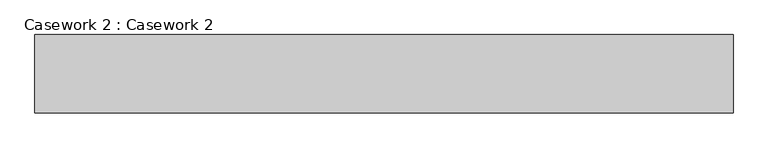
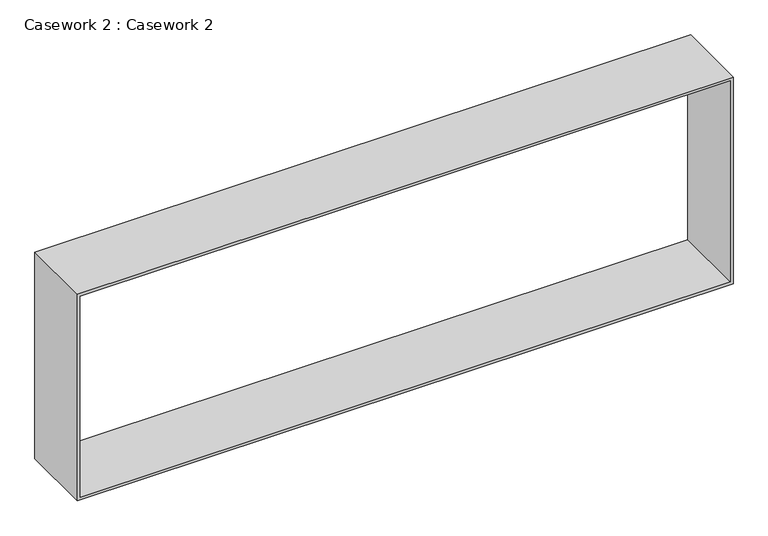
"""IFC4 building model written with IfcOpenShell, lengths in millimetres: furniture geometry, Casework 2 : Casework 2."""

from ifc_helpers import new_model, si_unit, frame, origin, place, context, project, spatial, polyline, outline, extrude, source, transform, mapped, element, save


def casework_2_casework_2_d1309b6c(model_context):
    return source(origin(), model_context, "Body", "SweptSolid", [
        extrude(outline(polyline([(2743.2, -50908.4551606), (914.4, -50908.4551606), (914.4, -45422.0551606), (2743.2, -45422.0551606), (2743.2, -50908.4551606)]), holes=[polyline([(2717.8, -50883.0551606), (2717.8, -45447.4551606), (939.8, -45447.4551606), (939.8, -50883.0551606), (2717.8, -50883.0551606)])]), frame((0.0, 287138.3720148, 0.0), z_axis=(0.0, 1.0, 0.0), x_axis=(0.0, 0.0, 1.0)), (0.0, 0.0, 1.0), 614.656204),
    ])


if __name__ == "__main__":
    model = new_model("IFC4")
    model_context = context("Model", 3, world=origin())
    ifc_project = project(units=[si_unit("LENGTHUNIT", "METRE", prefix="MILLI")], contexts=[model_context])
    site = spatial("IfcSite", under=ifc_project)
    building = spatial("IfcBuilding", under=site)
    placement = place(None, origin())
    casework_2_casework_2_shape = casework_2_casework_2_d1309b6c(model_context)
    element("IfcFurniture", 1, ObjectType="Casework 2 : Casework 2", at=placement, inside=building, context=model_context, shape_type="MappedRepresentation", body=[
        mapped(casework_2_casework_2_shape, transform((0.0, 0.0, 0.0), x_axis=(1.0, 0.0, 0.0), y_axis=(0.0, 1.0, 0.0), z_axis=(0.0, 0.0, 1.0))),
    ])
    save(model, "model.ifc")

# Revit data of these elements
# Element 1 (IfcFurniture, "Casework 2 : Casework 2")
#   Materials on its faces: "1.50\" ASPHALT SURFACE COURSE (E-0.3)"
# Materials
#   "1.50\" ASPHALT SURFACE COURSE (E-0.3)": class "Miscellaneous", colour RGB 164 164 164, transparency 0, Cost = 0
